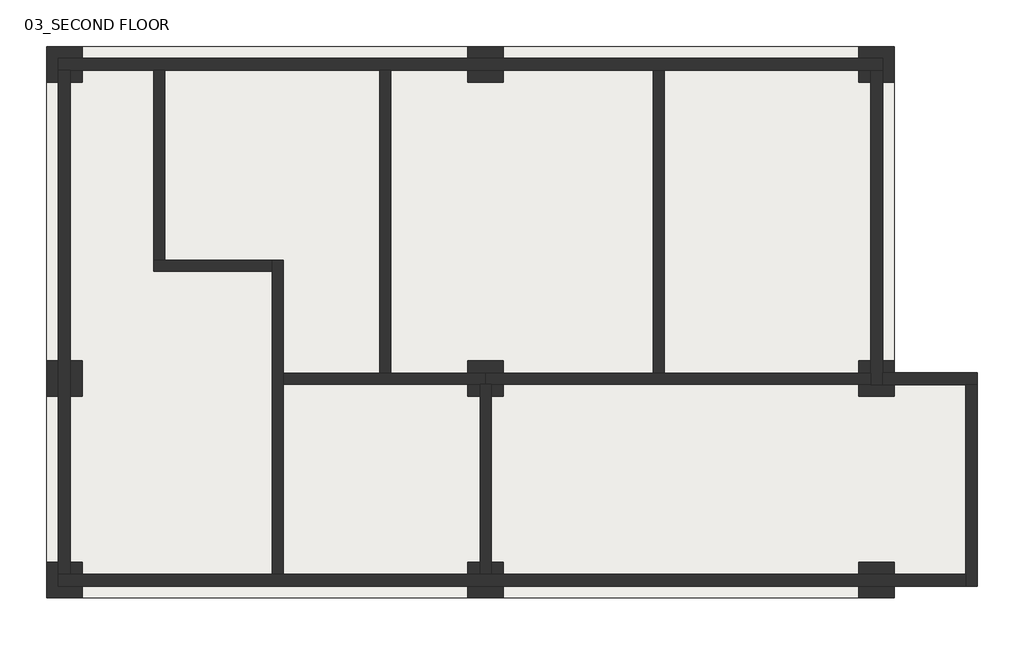
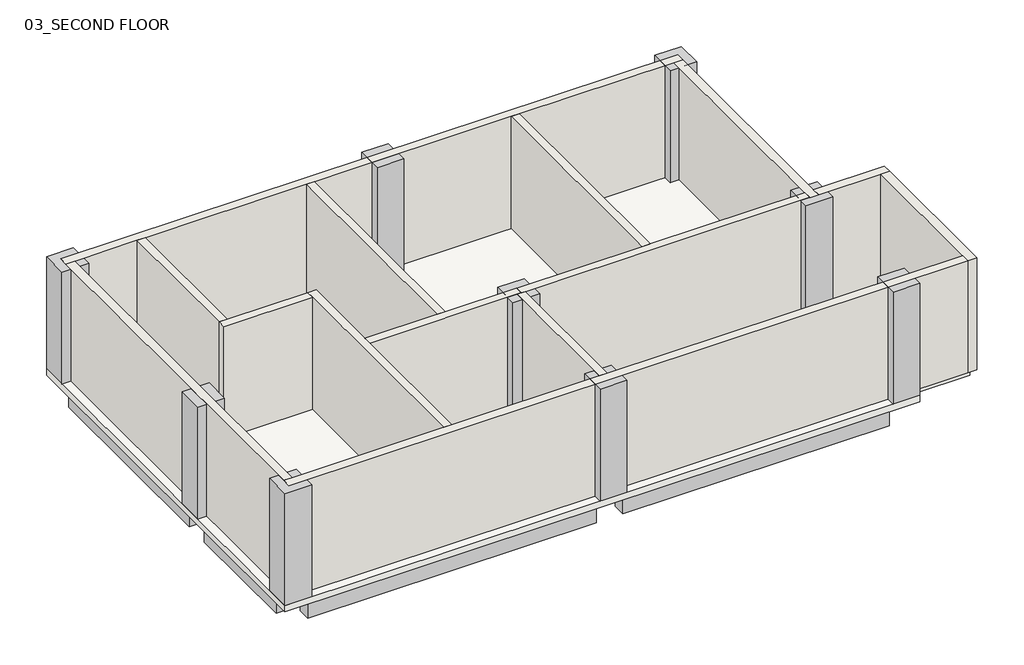
# One storey: 14 walls, 12 beams, 9 columns, 1 slab.
"""IFC4 building model written with IfcOpenShell, lengths in millimetres."""

from ifc_helpers import new_model, si_unit, frame, origin, place, context, project, spatial, polyline, outline, extrude, faceted_brep, element, save

model = new_model("IFC4")

# Units and contexts
model_context = context("Model", 3, world=origin())
ifc_project = project(units=[si_unit("LENGTHUNIT", "METRE", prefix="MILLI")], contexts=[model_context])

# Site, building, storey
site = spatial("IfcSite", under=ifc_project)
building = spatial("IfcBuilding", under=site)
storey = spatial("IfcBuildingStorey", under=building, Name="03_SECOND FLOOR", Elevation=5969.9618634)

# Beams
placement = place(None, origin())
element("IfcBeam", 1, ObjectType="RC Beam_Rectangular : H_SB_AR_S16_B300xH600", at=placement, inside=storey, context=model_context, shape_type="SweptSolid", body=[
    extrude(outline(polyline([(300.0, 1049.5208589), (300.0, 1349.5208589), (6800.0, 1349.5208589), (6800.0, 1049.5208589), (300.0, 1049.5208589)])), frame((0.0, 0.0, 5369.9618634), z_axis=(0.0, 0.0, 1.0), x_axis=(1.0, 0.0, 0.0)), (0.0, 0.0, 1.0), 450.0),
])
element("IfcBeam", 2, ObjectType="RC Beam_Rectangular : H_SB_AR_S16_B300xH600", at=placement, inside=storey, context=model_context, shape_type="SweptSolid", body=[
    extrude(outline(polyline([(7400.0, 1049.5208589), (7400.0, 1349.5208589), (13400.0, 1349.5208589), (13400.0, 1049.5208589), (7400.0, 1049.5208589)])), frame((0.0, 0.0, 5369.9618634), z_axis=(0.0, 0.0, 1.0), x_axis=(1.0, 0.0, 0.0)), (0.0, 0.0, 1.0), 450.0),
])
element("IfcBeam", 3, ObjectType="RC Beam_Rectangular : H_SB_AR_S16_B300xH600", at=placement, inside=storey, context=model_context, shape_type="SweptSolid", body=[
    extrude(outline(polyline([(300.0, 6349.5208589), (300.0, 6649.5208589), (6800.0, 6649.5208589), (6800.0, 6349.5208589), (300.0, 6349.5208589)])), frame((0.0, 0.0, 5369.9618634), z_axis=(0.0, 0.0, 1.0), x_axis=(1.0, 0.0, 0.0)), (0.0, 0.0, 1.0), 450.0),
])
element("IfcBeam", 4, ObjectType="RC Beam_Rectangular : H_SB_AR_S16_B300xH600", at=placement, inside=storey, context=model_context, shape_type="SweptSolid", body=[
    extrude(outline(polyline([(7400.0, 6349.5208589), (7400.0, 6649.5208589), (13400.0, 6649.5208589), (13400.0, 6349.5208589), (7400.0, 6349.5208589)])), frame((0.0, 0.0, 5369.9618634), z_axis=(0.0, 0.0, 1.0), x_axis=(1.0, 0.0, 0.0)), (0.0, 0.0, 1.0), 450.0),
])
element("IfcBeam", 5, ObjectType="RC Beam_Rectangular : H_SB_AR_S16_B300xH600", at=placement, inside=storey, context=model_context, shape_type="SweptSolid", body=[
    extrude(outline(polyline([(300.0, -2350.4791411), (300.0, -2050.4791411), (6800.0, -2050.4791411), (6800.0, -2350.4791411), (300.0, -2350.4791411)])), frame((0.0, 0.0, 5369.9618634), z_axis=(0.0, 0.0, 1.0), x_axis=(1.0, 0.0, 0.0)), (0.0, 0.0, 1.0), 450.0),
])
element("IfcBeam", 6, ObjectType="RC Beam_Rectangular : H_SB_AR_S16_B300xH600", at=placement, inside=storey, context=model_context, shape_type="SweptSolid", body=[
    extrude(outline(polyline([(7400.0, -2350.4791411), (7400.0, -2050.4791411), (13400.0, -2050.4791411), (13400.0, -2350.4791411), (7400.0, -2350.4791411)])), frame((0.0, 0.0, 5369.9618634), z_axis=(0.0, 0.0, 1.0), x_axis=(1.0, 0.0, 0.0)), (0.0, 0.0, 1.0), 450.0),
])
element("IfcBeam", 7, ObjectType="RC Beam_Rectangular : H_SB_AR_S16_B300xH600", at=placement, inside=storey, context=model_context, shape_type="SweptSolid", body=[
    extrude(outline(polyline([(-150.0, 899.5208589), (150.0, 899.5208589), (150.0, -1900.4791411), (-150.0, -1900.4791411), (-150.0, 899.5208589)])), frame((0.0, 0.0, 5369.9618634), z_axis=(0.0, 0.0, 1.0), x_axis=(1.0, 0.0, 0.0)), (0.0, 0.0, 1.0), 450.0),
])
element("IfcBeam", 8, ObjectType="RC Beam_Rectangular : H_SB_AR_S16_B300xH600", at=placement, inside=storey, context=model_context, shape_type="SweptSolid", body=[
    extrude(outline(polyline([(150.0, 1499.5208589), (-150.0, 1499.5208589), (-150.0, 6199.5208589), (150.0, 6199.5208589), (150.0, 1499.5208589)])), frame((0.0, 0.0, 5369.9618634), z_axis=(0.0, 0.0, 1.0), x_axis=(1.0, 0.0, 0.0)), (0.0, 0.0, 1.0), 450.0),
])
element("IfcBeam", 9, ObjectType="RC Beam_Rectangular : H_SB_AR_S16_B300xH600", at=placement, inside=storey, context=model_context, shape_type="SweptSolid", body=[
    extrude(outline(polyline([(6950.0, 899.5208589), (7250.0, 899.5208589), (7250.0, -1900.4791411), (6950.0, -1900.4791411), (6950.0, 899.5208589)])), frame((0.0, 0.0, 5369.9618634), z_axis=(0.0, 0.0, 1.0), x_axis=(1.0, 0.0, 0.0)), (0.0, 0.0, 1.0), 450.0),
])
element("IfcBeam", 10, ObjectType="RC Beam_Rectangular : H_SB_AR_S16_B300xH600", at=placement, inside=storey, context=model_context, shape_type="SweptSolid", body=[
    extrude(outline(polyline([(7250.0, 1499.5208589), (6950.0, 1499.5208589), (6950.0, 6199.5208589), (7250.0, 6199.5208589), (7250.0, 1499.5208589)])), frame((0.0, 0.0, 5369.9618634), z_axis=(0.0, 0.0, 1.0), x_axis=(1.0, 0.0, 0.0)), (0.0, 0.0, 1.0), 450.0),
])
element("IfcBeam", 11, ObjectType="RC Beam_Rectangular : H_SB_AR_S16_B300xH600", at=placement, inside=storey, context=model_context, shape_type="SweptSolid", body=[
    extrude(outline(polyline([(13550.0, 899.5208589), (13850.0, 899.5208589), (13850.0, -1900.4791411), (13550.0, -1900.4791411), (13550.0, 899.5208589)])), frame((0.0, 0.0, 5369.9618634), z_axis=(0.0, 0.0, 1.0), x_axis=(1.0, 0.0, 0.0)), (0.0, 0.0, 1.0), 450.0),
])
element("IfcBeam", 12, ObjectType="RC Beam_Rectangular : H_SB_AR_S16_B300xH600", at=placement, inside=storey, context=model_context, shape_type="SweptSolid", body=[
    extrude(outline(polyline([(13850.0, 1499.5208589), (13550.0, 1499.5208589), (13550.0, 6199.5208589), (13850.0, 6199.5208589), (13850.0, 1499.5208589)])), frame((0.0, 0.0, 5369.9618634), z_axis=(0.0, 0.0, 1.0), x_axis=(1.0, 0.0, 0.0)), (0.0, 0.0, 1.0), 450.0),
])

# Columns
element("IfcColumn", 13, ObjectType="RC_Column_Rectangular : H_SC_AR_S15_W600xL600", at=placement, inside=storey, context=model_context, shape_type="SweptSolid", body=[
    extrude(outline(polyline([(300.0, 1499.5208589), (300.0, 899.5208589), (-300.0, 899.5208589), (-300.0, 1499.5208589), (300.0, 1499.5208589)])), frame((0.0, 0.0, 5969.9618634), z_axis=(0.0, 0.0, 1.0), x_axis=(1.0, 0.0, 0.0)), (0.0, 0.0, 1.0), 2670.0),
])
element("IfcColumn", 14, ObjectType="RC_Column_Rectangular : H_SC_AR_S15_W600xL600", at=placement, inside=storey, context=model_context, shape_type="SweptSolid", body=[
    extrude(outline(polyline([(7400.0, 1499.5208589), (7400.0, 899.5208589), (6800.0, 899.5208589), (6800.0, 1499.5208589), (7400.0, 1499.5208589)])), frame((0.0, 0.0, 5969.9618634), z_axis=(0.0, 0.0, 1.0), x_axis=(1.0, 0.0, 0.0)), (0.0, 0.0, 1.0), 2670.0),
])
element("IfcColumn", 15, ObjectType="RC_Column_Rectangular : H_SC_AR_S15_W600xL600", at=placement, inside=storey, context=model_context, shape_type="SweptSolid", body=[
    extrude(outline(polyline([(14000.0, 1499.5208589), (14000.0, 899.5208589), (13400.0, 899.5208589), (13400.0, 1499.5208589), (14000.0, 1499.5208589)])), frame((0.0, 0.0, 5969.9618634), z_axis=(0.0, 0.0, 1.0), x_axis=(1.0, 0.0, 0.0)), (0.0, 0.0, 1.0), 2670.0),
])
element("IfcColumn", 16, ObjectType="RC_Column_Rectangular : H_SC_AR_S15_W600xL600", at=placement, inside=storey, context=model_context, shape_type="SweptSolid", body=[
    extrude(outline(polyline([(300.0, 6799.5208589), (300.0, 6199.5208589), (-300.0, 6199.5208589), (-300.0, 6799.5208589), (300.0, 6799.5208589)])), frame((0.0, 0.0, 5969.9618634), z_axis=(0.0, 0.0, 1.0), x_axis=(1.0, 0.0, 0.0)), (0.0, 0.0, 1.0), 2670.0),
])
element("IfcColumn", 17, ObjectType="RC_Column_Rectangular : H_SC_AR_S15_W600xL600", at=placement, inside=storey, context=model_context, shape_type="SweptSolid", body=[
    extrude(outline(polyline([(7400.0, 6799.5208589), (7400.0, 6199.5208589), (6800.0, 6199.5208589), (6800.0, 6799.5208589), (7400.0, 6799.5208589)])), frame((0.0, 0.0, 5969.9618634), z_axis=(0.0, 0.0, 1.0), x_axis=(1.0, 0.0, 0.0)), (0.0, 0.0, 1.0), 2670.0),
])
element("IfcColumn", 18, ObjectType="RC_Column_Rectangular : H_SC_AR_S15_W600xL600", at=placement, inside=storey, context=model_context, shape_type="SweptSolid", body=[
    extrude(outline(polyline([(14000.0, 6799.5208589), (14000.0, 6199.5208589), (13400.0, 6199.5208589), (13400.0, 6799.5208589), (14000.0, 6799.5208589)])), frame((0.0, 0.0, 5969.9618634), z_axis=(0.0, 0.0, 1.0), x_axis=(1.0, 0.0, 0.0)), (0.0, 0.0, 1.0), 2670.0),
])
element("IfcColumn", 19, ObjectType="RC_Column_Rectangular : H_SC_AR_S15_W600xL600", at=placement, inside=storey, context=model_context, shape_type="SweptSolid", body=[
    extrude(outline(polyline([(300.0, -1900.4791411), (300.0, -2500.4791411), (-300.0, -2500.4791411), (-300.0, -1900.4791411), (300.0, -1900.4791411)])), frame((0.0, 0.0, 5969.9618634), z_axis=(0.0, 0.0, 1.0), x_axis=(1.0, 0.0, 0.0)), (0.0, 0.0, 1.0), 2670.0),
])
element("IfcColumn", 20, ObjectType="RC_Column_Rectangular : H_SC_AR_S15_W600xL600", at=placement, inside=storey, context=model_context, shape_type="SweptSolid", body=[
    extrude(outline(polyline([(7400.0, -1900.4791411), (7400.0, -2500.4791411), (6800.0, -2500.4791411), (6800.0, -1900.4791411), (7400.0, -1900.4791411)])), frame((0.0, 0.0, 5969.9618634), z_axis=(0.0, 0.0, 1.0), x_axis=(1.0, 0.0, 0.0)), (0.0, 0.0, 1.0), 2670.0),
])
element("IfcColumn", 21, ObjectType="RC_Column_Rectangular : H_SC_AR_S15_W600xL600", at=placement, inside=storey, context=model_context, shape_type="SweptSolid", body=[
    extrude(outline(polyline([(14000.0, -1900.4791411), (14000.0, -2500.4791411), (13400.0, -2500.4791411), (13400.0, -1900.4791411), (14000.0, -1900.4791411)])), frame((0.0, 0.0, 5969.9618634), z_axis=(0.0, 0.0, 1.0), x_axis=(1.0, 0.0, 0.0)), (0.0, 0.0, 1.0), 2670.0),
])

# Slab
element("IfcSlab", 22, ObjectType="H_FL_AR_S17_RC Slab T150", at=placement, inside=storey, context=model_context, shape_type="SweptSolid", body=[
    extrude(outline(polyline([(14000.0, 1199.5208589), (15300.0, 1199.5208589), (15300.0, -2200.4791411), (14000.0, -2200.4791411), (14000.0, -2500.4791411), (-300.0, -2500.4791411), (-300.0, 6799.5208589), (14000.0, 6799.5208589), (14000.0, 1199.5208589)])), frame((0.0, 0.0, 5819.9618634), z_axis=(0.0, 0.0, 1.0), x_axis=(1.0, 0.0, 0.0)), (0.0, 0.0, 1.0), 150.0),
])

# Walls
element("IfcWall", 23, ObjectType="H_WA_AR_B02_Ext Wall_RC T200", at=placement, inside=storey, context=model_context, shape_type="Brep", body=[
    faceted_brep([(-100.0, 6399.5208589, 5969.9618634), (100.0, 6399.5208589, 5969.9618634), (1506.0, 6399.5208589, 5969.9618634), (1690.0, 6399.5208589, 5969.9618634), (5320.5, 6399.5208589, 5969.9618634), (5504.5, 6399.5208589, 5969.9618634), (9935.0, 6399.5208589, 5969.9618634), (10119.0, 6399.5208589, 5969.9618634), (13600.0, 6399.5208589, 5969.9618634), (13800.0, 6399.5208589, 5969.9618634), (13800.0, 6399.5208589, 8639.9618634), (13600.0, 6399.5208589, 8639.9618634), (10119.0, 6399.5208589, 8639.9618634), (9935.0, 6399.5208589, 8639.9618634), (5504.5, 6399.5208589, 8639.9618634), (5320.5, 6399.5208589, 8639.9618634), (1690.0, 6399.5208589, 8639.9618634), (1506.0, 6399.5208589, 8639.9618634), (100.0, 6399.5208589, 8639.9618634), (-100.0, 6399.5208589, 8639.9618634), (-100.0, 6599.5208589, 5969.9618634), (-100.0, 6599.5208589, 8639.9618634), (13800.0, 6599.5208589, 8639.9618634), (13800.0, 6599.5208589, 5969.9618634)], [[[0, 1, 2, 3, 4, 5, 6, 7, 8, 9, 10, 11, 12, 13, 14, 15, 16, 17, 18, 19]], [[20, 21, 22, 23]], [[9, 8, 7, 6, 5, 4, 3, 2, 1, 0, 20, 23]], [[19, 18, 17, 16, 15, 14, 13, 12, 11, 10, 22, 21]], [[10, 9, 23, 22]], [[0, 19, 21, 20]]]),
])
element("IfcWall", 24, ObjectType="H_WA_AR_B02_Ext Wall_RC T200", at=placement, inside=storey, context=model_context, shape_type="Brep", body=[
    faceted_brep([(13600.0, 6399.5208589, 5969.9618634), (13600.0, 1286.5208589, 5969.9618634), (13600.0, 1102.5208589, 5969.9618634), (13600.0, 1099.5208589, 5969.9618634), (13600.0, 1099.5208589, 8639.9618634), (13600.0, 1102.5208589, 8639.9618634), (13600.0, 1286.5208589, 8639.9618634), (13600.0, 6399.5208589, 8639.9618634), (13800.0, 6399.5208589, 5969.9618634), (13800.0, 6399.5208589, 8639.9618634), (13800.0, 1299.5208589, 8639.9618634), (13800.0, 1099.5208589, 8639.9618634), (13800.0, 1099.5208589, 5969.9618634), (13800.0, 1299.5208589, 5969.9618634)], [[[0, 1, 2, 3, 4, 5, 6, 7]], [[8, 9, 10, 11, 12, 13]], [[3, 2, 1, 0, 8, 13, 12]], [[7, 6, 5, 4, 11, 10, 9]], [[0, 7, 9, 8]], [[4, 3, 12, 11]]]),
])
element("IfcWall", 25, ObjectType="H_WA_AR_B02_Ext Wall_RC T200", at=placement, inside=storey, context=model_context, shape_type="Brep", body=[
    faceted_brep([(13800.0, 1099.5208589, 5969.9618634), (15200.0, 1099.5208589, 5969.9618634), (15400.0, 1099.5208589, 5969.9618634), (15400.0, 1099.5208589, 8639.9618634), (15200.0, 1099.5208589, 8639.9618634), (13800.0, 1099.5208589, 8639.9618634), (13800.0, 1299.5208589, 5969.9618634), (13800.0, 1299.5208589, 8639.9618634), (15400.0, 1299.5208589, 8639.9618634), (15400.0, 1299.5208589, 5969.9618634)], [[[0, 1, 2, 3, 4, 5]], [[6, 7, 8, 9]], [[2, 1, 0, 6, 9]], [[5, 4, 3, 8, 7]], [[0, 5, 7, 6]], [[3, 2, 9, 8]]]),
])
element("IfcWall", 26, ObjectType="H_WA_AR_B02_Ext Wall_RC T200", at=placement, inside=storey, context=model_context, shape_type="Brep", body=[
    faceted_brep([(15200.0, 1099.5208589, 5969.9618634), (15200.0, -2100.4791411, 5969.9618634), (15200.0, -2300.4791411, 5969.9618634), (15200.0, -2300.4791411, 8639.9618634), (15200.0, -2100.4791411, 8639.9618634), (15200.0, 1099.5208589, 8639.9618634), (15400.0, 1099.5208589, 5969.9618634), (15400.0, 1099.5208589, 8639.9618634), (15400.0, -2300.4791411, 8639.9618634), (15400.0, -2300.4791411, 5969.9618634)], [[[0, 1, 2, 3, 4, 5]], [[6, 7, 8, 9]], [[2, 1, 0, 6, 9]], [[5, 4, 3, 8, 7]], [[0, 5, 7, 6]], [[3, 2, 9, 8]]]),
])
element("IfcWall", 27, ObjectType="H_WA_AR_B02_Ext Wall_RC T200", at=placement, inside=storey, context=model_context, shape_type="Brep", body=[
    faceted_brep([(15200.0, -2100.4791411, 5969.9618634), (7197.0, -2100.4791411, 5969.9618634), (7013.0, -2100.4791411, 5969.9618634), (3690.0, -2100.4791411, 5969.9618634), (3506.0, -2100.4791411, 5969.9618634), (100.0, -2100.4791411, 5969.9618634), (-100.0, -2100.4791411, 5969.9618634), (-100.0, -2100.4791411, 8639.9618634), (100.0, -2100.4791411, 8639.9618634), (3506.0, -2100.4791411, 8639.9618634), (3690.0, -2100.4791411, 8639.9618634), (7013.0, -2100.4791411, 8639.9618634), (7197.0, -2100.4791411, 8639.9618634), (15200.0, -2100.4791411, 8639.9618634), (15200.0, -2300.4791411, 5969.9618634), (15200.0, -2300.4791411, 8639.9618634), (-100.0, -2300.4791411, 8639.9618634), (-100.0, -2300.4791411, 5969.9618634)], [[[0, 1, 2, 3, 4, 5, 6, 7, 8, 9, 10, 11, 12, 13]], [[14, 15, 16, 17]], [[6, 5, 4, 3, 2, 1, 0, 14, 17]], [[13, 12, 11, 10, 9, 8, 7, 16, 15]], [[0, 13, 15, 14]], [[7, 6, 17, 16]]]),
])
element("IfcWall", 28, ObjectType="H_WA_AR_B02_Ext Wall_RC T200", at=placement, inside=storey, context=model_context, shape_type="SweptSolid", body=[
    extrude(outline(polyline([(100.0, 6399.5208589), (100.0, -2100.4791411), (-100.0, -2100.4791411), (-100.0, 6399.5208589), (100.0, 6399.5208589)])), frame((0.0, 0.0, 5969.9618634), z_axis=(0.0, 0.0, 1.0), x_axis=(1.0, 0.0, 0.0)), (0.0, 0.0, 1.0), 2670.0),
])
element("IfcWall", 29, ObjectType="H_WA_AR_B02_Int Wall_Block T150", at=placement, inside=storey, context=model_context, shape_type="Brep", body=[
    faceted_brep([(7197.0, -2100.4791411, 5969.9618634), (7197.0, 1102.5208589, 5969.9618634), (7197.0, 1102.5208589, 8639.9618634), (7197.0, -2100.4791411, 8639.9618634), (7013.0, -2100.4791411, 5969.9618634), (7013.0, -2100.4791411, 8639.9618634), (7013.0, 1102.5208589, 8639.9618634), (7013.0, 1102.5208589, 5969.9618634), (7105.0, 1102.5208589, 5969.9618634), (7105.0, 1102.5208589, 8639.9618634)], [[[0, 1, 2, 3]], [[4, 5, 6, 7]], [[1, 0, 4, 7, 8]], [[3, 2, 9, 6, 5]], [[0, 3, 5, 4]], [[2, 1, 8, 7, 6, 9]]]),
])
element("IfcWall", 30, ObjectType="H_WA_AR_B02_Int Wall_Block T150", at=placement, inside=storey, context=model_context, shape_type="Brep", body=[
    faceted_brep([(7105.0, 1102.5208589, 5969.9618634), (7197.0, 1102.5208589, 5969.9618634), (13600.0, 1102.5208589, 5969.9618634), (13600.0, 1102.5208589, 8639.9618634), (7197.0, 1102.5208589, 8639.9618634), (7105.0, 1102.5208589, 8639.9618634), (7105.0, 1286.5208589, 5969.9618634), (7105.0, 1286.5208589, 8639.9618634), (9935.0, 1286.5208589, 8639.9618634), (10119.0, 1286.5208589, 8639.9618634), (13600.0, 1286.5208589, 8639.9618634), (13600.0, 1286.5208589, 5969.9618634), (10119.0, 1286.5208589, 5969.9618634), (9935.0, 1286.5208589, 5969.9618634)], [[[0, 1, 2, 3, 4, 5]], [[6, 7, 8, 9, 10, 11, 12, 13]], [[2, 1, 0, 6, 13, 12, 11]], [[5, 4, 3, 10, 9, 8, 7]], [[0, 5, 7, 6]], [[3, 2, 11, 10]]]),
])
element("IfcWall", 31, ObjectType="H_WA_AR_B02_Int Wall_Block T150", at=placement, inside=storey, context=model_context, shape_type="Brep", body=[
    faceted_brep([(3690.0, -2100.4791411, 5969.9618634), (3690.0, 1107.5208589, 5969.9618634), (3690.0, 1291.5208589, 5969.9618634), (3690.0, 3196.5208589, 5969.9618634), (3690.0, 3196.5208589, 8639.9618634), (3690.0, 1291.5208589, 8639.9618634), (3690.0, 1107.5208589, 8639.9618634), (3690.0, -2100.4791411, 8639.9618634), (3506.0, -2100.4791411, 5969.9618634), (3506.0, -2100.4791411, 8639.9618634), (3506.0, 3012.5208589, 8639.9618634), (3506.0, 3196.5208589, 8639.9618634), (3506.0, 3196.5208589, 5969.9618634), (3506.0, 3012.5208589, 5969.9618634)], [[[0, 1, 2, 3, 4, 5, 6, 7]], [[8, 9, 10, 11, 12, 13]], [[3, 2, 1, 0, 8, 13, 12]], [[7, 6, 5, 4, 11, 10, 9]], [[0, 7, 9, 8]], [[4, 3, 12, 11]]]),
])
element("IfcWall", 32, ObjectType="H_WA_AR_B02_Int Wall_Block T150", at=placement, inside=storey, context=model_context, shape_type="Brep", body=[
    faceted_brep([(3506.0, 3196.5208589, 5969.9618634), (1690.0, 3196.5208589, 5969.9618634), (1506.0, 3196.5208589, 5969.9618634), (1506.0, 3196.5208589, 8639.9618634), (1690.0, 3196.5208589, 8639.9618634), (3506.0, 3196.5208589, 8639.9618634), (3506.0, 3012.5208589, 5969.9618634), (3506.0, 3012.5208589, 8639.9618634), (1506.0, 3012.5208589, 8639.9618634), (1506.0, 3012.5208589, 5969.9618634)], [[[0, 1, 2, 3, 4, 5]], [[6, 7, 8, 9]], [[2, 1, 0, 6, 9]], [[5, 4, 3, 8, 7]], [[0, 5, 7, 6]], [[3, 2, 9, 8]]]),
])
element("IfcWall", 33, ObjectType="H_WA_AR_B02_Int Wall_Block T150", at=placement, inside=storey, context=model_context, shape_type="SweptSolid", body=[
    extrude(outline(polyline([(1690.0, 6399.5208589), (1690.0, 3196.5208589), (1506.0, 3196.5208589), (1506.0, 6399.5208589), (1690.0, 6399.5208589)])), frame((0.0, 0.0, 5969.9618634), z_axis=(0.0, 0.0, 1.0), x_axis=(1.0, 0.0, 0.0)), (0.0, 0.0, 1.0), 2670.0),
])
element("IfcWall", 34, ObjectType="H_WA_AR_B02_Int Wall_Block T150", at=placement, inside=storey, context=model_context, shape_type="Brep", body=[
    faceted_brep([(7100.0, 1291.5208589, 5969.9618634), (5504.5, 1291.5208589, 5969.9618634), (5320.5, 1291.5208589, 5969.9618634), (3690.0, 1291.5208589, 5969.9618634), (3690.0, 1291.5208589, 8639.9618634), (5320.5, 1291.5208589, 8639.9618634), (5504.5, 1291.5208589, 8639.9618634), (7100.0, 1291.5208589, 8639.9618634), (7100.0, 1107.5208589, 5969.9618634), (7100.0, 1107.5208589, 8639.9618634), (3690.0, 1107.5208589, 8639.9618634), (3690.0, 1107.5208589, 5969.9618634)], [[[0, 1, 2, 3, 4, 5, 6, 7]], [[8, 9, 10, 11]], [[3, 2, 1, 0, 8, 11]], [[7, 6, 5, 4, 10, 9]], [[0, 7, 9, 8]], [[4, 3, 11, 10]]]),
])
element("IfcWall", 35, ObjectType="H_WA_AR_B02_Int Wall_Block T150", at=placement, inside=storey, context=model_context, shape_type="SweptSolid", body=[
    extrude(outline(polyline([(5504.5, 6399.5208589), (5504.5, 1291.5208589), (5320.5, 1291.5208589), (5320.5, 6399.5208589), (5504.5, 6399.5208589)])), frame((0.0, 0.0, 5969.9618634), z_axis=(0.0, 0.0, 1.0), x_axis=(1.0, 0.0, 0.0)), (0.0, 0.0, 1.0), 2670.0),
])
element("IfcWall", 36, ObjectType="H_WA_AR_B02_Int Wall_Block T150", at=placement, inside=storey, context=model_context, shape_type="SweptSolid", body=[
    extrude(outline(polyline([(10119.0, 6399.5208589), (10119.0, 1286.5208589), (9935.0, 1286.5208589), (9935.0, 6399.5208589), (10119.0, 6399.5208589)])), frame((0.0, 0.0, 5969.9618634), z_axis=(0.0, 0.0, 1.0), x_axis=(1.0, 0.0, 0.0)), (0.0, 0.0, 1.0), 2670.0),
])

save(model, "model.ifc")

# Revit data of these elements
# Type "RC Beam_Rectangular : H_SB_AR_S16_B300xH600"
#   중앙부 하부근 = ""
#   중앙부 상부근 = ""
#   중앙부 보조근 = ""
#   중앙부 늑근 = ""
#   외단부 하부근 = ""
#   외단부 상부근 = ""
#   외단부 보조근 = ""
#   외단부 늑근 = ""
#   부호 = "TG3"
#   내단부 하부근 = ""
#   내단부 상부근 = ""
#   내단부 보조근 = ""
#   내단부 늑근 = ""
#   ALL 하부근 = "3-D20"
#   ALL 상부근 = "3-D20"
#   ALL 보조근 = ""
#   ALL 늑근 = "2-D10 @120"
#   Width = 300 mm
#   Height = 600 mm
#   Length [instance default] = 1524 mm
#   b = 300 mm
#   h = 600 mm
#   hec_material3 [instance default] = none
#   hec_material2 [instance default] = none
#   hec_material1 [instance default] = none
#   Structural Material [instance default] = none
#   Assembly Code = ""
# Type "RC_Column_Rectangular : H_SC_AR_S15_W600xL600"
#   Width = 600 mm
#   Length = 600 mm
#   hec_material3 [instance default] = none
#   hec_material2 [instance default] = none
#   hec_material1 [instance default] = none
#   Structural Material [instance default] = none
#   Description = (empty or 0)
# Type "H_FL_AR_S17_RC Slab T150"
#   Keynote = ""
#   Type Comments = ""
#   Description = ""
#   Function = 1
#   Layers, outside or top first: 150 mm no material (function 1)
# Type "H_WA_AR_B02_Ext Wall_RC T200"
#   Type Comments = ""
#   Layers, outside or top first: 0 mm no material (function 100); 0 mm no material (function 100); 200 mm no material (function 1); 0 mm no material (function 100); 0 mm no material (function 100); 0 mm no material (function 100)
# Type "H_WA_AR_B02_Int Wall_Block T150"
#   Type Comments = ""
#   Layers, outside or top first: 0 mm no material (function 100); 12 mm no material (function 2); 150 mm no material (function 1); 12 mm no material (function 2); 10 mm no material (function 5)
# Elements 1, 2, 3, 4, 5, 6, 7, 8, 9, 10, 11, 12 (IfcBeam, "RC Beam_Rectangular : H_SB_AR_S16_B300xH600")
#   Comments = ""
#   hec_material3 = none
#   hec_material2 = none
#   hec_material1 = none
#   Structural Material = none
#   Phase Created = New Construction
# Elements 13, 14, 15, 16, 17, 18, 19, 20, 21 (IfcColumn, "RC_Column_Rectangular : H_SC_AR_S15_W600xL600")
#   Comments = ""
#   hec_material3 = none
#   hec_material2 = none
#   hec_material1 = none
#   Structural Material = none
#   Phase Created = New Construction
# Element 22 (IfcSlab, "H_FL_AR_S17_RC Slab T150")
#   Height Offset From Level = 0 mm
#   Phase Created = New Construction
#   Materials on its faces: "Default Floor"
# Elements 23, 24, 25, 26, 27, 28 (IfcWall, "H_WA_AR_B02_Ext Wall_RC T200")
#   Top Offset = 0 mm
#   Base Offset = 0 mm
#   wall height = 2670 mm
#   Phase Created = New Construction
#   Base Constraint = 03_SECOND FLOOR
#   Top Constraint = 04_THIRD FLOOR
#   Materials on its faces: "Default Wall"
# Elements 29, 30, 31, 32, 33, 34, 35, 36 (IfcWall, "H_WA_AR_B02_Int Wall_Block T150")
#   Top Offset = 0 mm
#   Base Offset = 0 mm
#   wall height = 2670 mm
#   Phase Created = New Construction
#   Base Constraint = 03_SECOND FLOOR
#   Top Constraint = 04_THIRD FLOOR
#   Materials on its faces: "Default Wall"
# Materials
#   "Default Floor": class "Miscellaneous", colour RGB 80 80 80, transparency 0
#   "Default Wall": class "Miscellaneous", colour RGB 80 80 80, transparency 0
# Room at (11202.5, -500.479) mm, phase "New Construction", upper level "04_THIRD FLOOR", upper offset 1000 mm, lower offset -1000 mm
#   Comments = ""
#   Number = "134"
#   Name = "STAIRS"
# Room at (1799, 2149.521) mm, phase "New Construction", upper level "04_THIRD FLOOR", upper offset 1000 mm, lower offset -1000 mm
#   Comments = ""
#   Number = "135"
#   Name = "CARBONACEOUS FIRE ROOM"
# Room at (5351.5, -500.479) mm, phase "New Construction", upper level "04_THIRD FLOOR", upper offset 1000 mm, lower offset -1000 mm
#   Comments = ""
#   Number = "136"
#   Name = "TECHNICAL TOWER"
# Room at (3505.25, 3849.521) mm, phase "New Construction", upper level "04_THIRD FLOOR", upper offset 1000 mm, lower offset -1000 mm
#   Comments = ""
#   Number = "137"
#   Name = "SMOKE ROOM"
# Room at (7719.75, 3847.021) mm, phase "New Construction", upper level "04_THIRD FLOOR", upper offset 1000 mm, lower offset -1000 mm
#   Comments = ""
#   Number = "138"
#   Name = "LPG FIRE ROOM"
# Room at (11863.5, 3847.021) mm, phase "New Construction", upper level "04_THIRD FLOOR", upper offset 1000 mm, lower offset -1000 mm
#   Comments = ""
#   Number = "139"
#   Name = "LOBBY"
